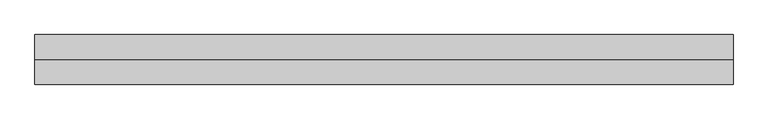
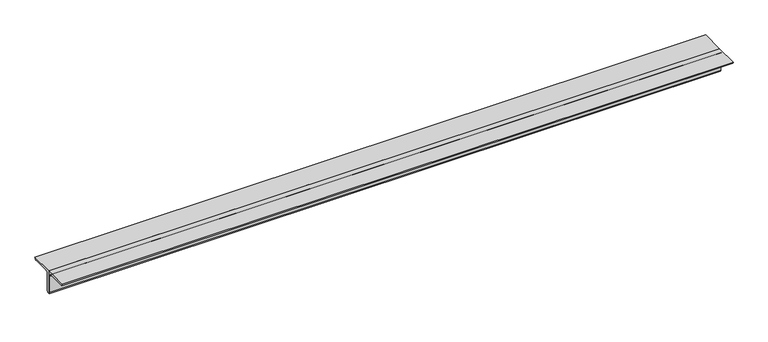
"""IFC4 building model written with IfcOpenShell, lengths in millimetres: member geometry, 0123_Steel Framing_2Ls-KSD3502 : H_SB_AR_S03_2Ls-130x130x12_HBR4."""

import ifcopenshell
import ifcopenshell.guid

model = None  # the IFC model being written
_history = None  # IfcOwnerHistory: only IFC2X3 demands one
_inside = {}  # id of a spatial element -> (the spatial element, [elements in it])
_under = {}  # id of a project, library or spatial element -> (it, [spatial elements below it])
_declared = {}  # id of a project -> (the project, [libraries it declares])
_typed = {}  # id of a type object -> (the type object, [elements of that type])
_made_of = {}  # id of a material, layer set ... -> (it, [elements and type objects made of it])


def new_model(schema):
    """Start an empty IFC model of exactly this schema.

    Asked for "IFC4X3", IfcOpenShell would pick the latest addendum, in which some entities
    have other attributes; the version numbers below select the first issue.
    IFC2X3 requires an IfcOwnerHistory on every rooted entity: one is made here for all.
    """
    global model, _history
    if schema == "IFC4X3":
        model = ifcopenshell.file(schema_version=(4, 3, 0, 0))
    else:
        model = ifcopenshell.file(schema=schema)
    _inside.clear()
    _under.clear()
    _declared.clear()
    _typed.clear()
    _made_of.clear()
    _history = None
    if model.schema == "IFC2X3":
        org = make("IfcOrganization", Name="unknown")
        user = make(
            "IfcPersonAndOrganization",
            ThePerson=make("IfcPerson", FamilyName="unknown"),
            TheOrganization=org,
        )
        app = make(
            "IfcApplication",
            ApplicationDeveloper=org,
            Version="unknown",
            ApplicationFullName="unknown",
            ApplicationIdentifier="unknown",
        )
        _history = make(
            "IfcOwnerHistory",
            OwningUser=user,
            OwningApplication=app,
            ChangeAction="ADDED",
            CreationDate=0,
        )
    return model


def make(cls, **values):
    """One entity of the class cls with the attributes given. An attribute that is None is left unset."""
    return model.create_entity(
        cls, **{name: value for name, value in values.items() if value is not None}
    )


def rooted(cls, **values):
    """An entity with a GlobalId (a new one), such as an element, a storey or a relation."""
    return make(cls, GlobalId=ifcopenshell.guid.new(), OwnerHistory=_history, **values)


def si_unit(unit_type, name, prefix=None):
    """IfcSIUnit, for example si_unit("LENGTHUNIT", "METRE", prefix="MILLI")."""
    return make("IfcSIUnit", UnitType=unit_type, Prefix=prefix, Name=name)


def assignment(units):
    """IfcUnitAssignment: the units of a project."""
    return None if units is None else make("IfcUnitAssignment", Units=units)


def point(xyz):
    """IfcCartesianPoint."""
    return None if xyz is None else make("IfcCartesianPoint", Coordinates=xyz)


def direction(xyz):
    """IfcDirection."""
    return None if xyz is None else make("IfcDirection", DirectionRatios=xyz)


def frame(location, z_axis=None, x_axis=None):
    """IfcAxis2Placement3D, a coordinate frame: its origin and axes. An axis left out is left unset."""
    return make(
        "IfcAxis2Placement3D",
        Location=point(location),
        Axis=direction(z_axis),
        RefDirection=direction(x_axis),
    )


def frame_2d(location, x_axis=None):
    """IfcAxis2Placement2D, a coordinate frame in the plane: its origin and x axis."""
    return make(
        "IfcAxis2Placement2D", Location=point(location), RefDirection=direction(x_axis)
    )


def origin():
    """The frame at (0, 0, 0) with its axes left unset."""
    return frame((0.0, 0.0, 0.0))


def place(relative_to, where):
    """IfcLocalPlacement: puts the frame where relative to a parent placement (None: the world)."""
    return make(
        "IfcLocalPlacement", PlacementRelTo=relative_to, RelativePlacement=where
    )


def context(
    kind, dimensions, precision=None, world=None, true_north=None, identifier=None
):
    """IfcGeometricRepresentationContext, for example the 3D "Model" context."""
    return make(
        "IfcGeometricRepresentationContext",
        ContextIdentifier=identifier,
        ContextType=kind,
        CoordinateSpaceDimension=dimensions,
        Precision=precision,
        WorldCoordinateSystem=world,
        TrueNorth=true_north,
    )


def project(units=None, contexts=None):
    """IfcProject with its units and contexts."""
    return rooted(
        "IfcProject",
        Name="project",
        RepresentationContexts=contexts,
        UnitsInContext=assignment(units),
    )


def spatial(cls, under=None, at=None, **own):
    """A site, building, storey or space (cls), placed at a placement, below another one or the project."""
    s = rooted(cls, ObjectPlacement=at, **own)
    if under is not None:
        _under.setdefault(under.id(), (under, []))[1].append(s)
    return s


def polyline(points):
    """IfcPolyline through the points."""
    return make("IfcPolyline", Points=[point(p) for p in points])


def circle_curve(where, radius):
    """IfcCircle in the frame where."""
    return make("IfcCircle", Position=where, Radius=radius)


def trimmed(basis, trim1, trim2, sense, master):
    """IfcTrimmedCurve: the piece of a basis curve between two trims."""
    return make(
        "IfcTrimmedCurve",
        BasisCurve=basis,
        Trim1=trim1,
        Trim2=trim2,
        SenseAgreement=sense,
        MasterRepresentation=master,
    )


def segment(curve, same_sense, transition):
    """IfcCompositeCurveSegment."""
    return make(
        "IfcCompositeCurveSegment",
        Transition=transition,
        SameSense=same_sense,
        ParentCurve=curve,
    )


def composite_curve(segments, self_intersect=None):
    """IfcCompositeCurve: segments joined end to end."""
    return make("IfcCompositeCurve", Segments=segments, SelfIntersect=self_intersect)


def outline(outer, holes=None, kind="AREA"):
    """IfcArbitraryClosedProfileDef: a profile drawn as a closed curve; with holes, ...WithVoids."""
    if holes is None:
        return make("IfcArbitraryClosedProfileDef", ProfileType=kind, OuterCurve=outer)
    return make(
        "IfcArbitraryProfileDefWithVoids",
        ProfileType=kind,
        OuterCurve=outer,
        InnerCurves=holes,
    )


def extrude(swept, where, along, depth):
    """IfcExtrudedAreaSolid: the profile swept, set in the frame where, extruded along a direction by depth."""
    return make(
        "IfcExtrudedAreaSolid",
        SweptArea=swept,
        Position=where,
        ExtrudedDirection=direction(along),
        Depth=depth,
    )


def shape(context_of_items, identifier, shape_type, items):
    """IfcShapeRepresentation: the items that make up one representation, for example the "Body"."""
    return make(
        "IfcShapeRepresentation",
        ContextOfItems=context_of_items,
        RepresentationIdentifier=identifier,
        RepresentationType=shape_type,
        Items=items,
    )


def source(mapping_origin, context_of_items, identifier, shape_type, items):
    """IfcRepresentationMap: a shape defined once, which mapped items show again and again."""
    return make(
        "IfcRepresentationMap",
        MappingOrigin=mapping_origin,
        MappedRepresentation=shape(context_of_items, identifier, shape_type, items),
    )


def transform(
    local_origin,
    x_axis=None,
    y_axis=None,
    z_axis=None,
    scale=None,
    scale2=None,
    scale3=None,
    uniform=True,
):
    """IfcCartesianTransformationOperator3D, or its non-uniform kind. x_axis, y_axis, z_axis: its Axis1, 2, 3."""
    if uniform:
        return make(
            "IfcCartesianTransformationOperator3D",
            Axis1=direction(x_axis),
            Axis2=direction(y_axis),
            LocalOrigin=point(local_origin),
            Scale=scale,
            Axis3=direction(z_axis),
        )
    return make(
        "IfcCartesianTransformationOperator3DnonUniform",
        Axis1=direction(x_axis),
        Axis2=direction(y_axis),
        LocalOrigin=point(local_origin),
        Scale=scale,
        Axis3=direction(z_axis),
        Scale2=scale2,
        Scale3=scale3,
    )


def mapped(mapping_source, mapping_target):
    """IfcMappedItem: shows the shape of a source again, moved by a transform."""
    return make(
        "IfcMappedItem", MappingSource=mapping_source, MappingTarget=mapping_target
    )


def made_of(thing, what):
    """Note that an element or type object is made of a material, layer set ...; save() writes the relation."""
    if what is not None:
        _made_of.setdefault(what.id(), (what, []))[1].append(thing)
    return thing


def element(
    cls,
    number,
    at=None,
    inside=None,
    cuts=None,
    type_object=None,
    material=None,
    context=None,
    identifier="Body",
    shape_type=None,
    held_by="IfcProductDefinitionShape",
    body=None,
    shapes=None,
    **own,
):
    """One element of the class cls, such as IfcWall. Its Tag is "e" and its number.

    at: its placement. inside: the storey or other place that contains it. cuts: it is an
    opening in that element (IfcRelVoidsElement). A single representation is given by context,
    identifier, shape_type and body (its items); several are given by shapes. held_by: the class
    of the entity that holds the representations. save() writes the other relations.
    """
    e = rooted(cls, Tag="e%d" % number, ObjectPlacement=at, **own)
    if body is not None:
        shapes = [shape(context, identifier, shape_type, body)]
    if shapes is not None:
        e.Representation = make(held_by, Representations=shapes)
    if inside is not None:
        _inside.setdefault(inside.id(), (inside, []))[1].append(e)
    if cuts is not None:
        rooted(
            "IfcRelVoidsElement", RelatingBuildingElement=cuts, RelatedOpeningElement=e
        )
    if type_object is not None:
        _typed.setdefault(type_object.id(), (type_object, []))[1].append(e)
    return made_of(e, material)


def aggregate(whole, parts):
    """IfcRelAggregates: a whole, such as a stair, and the parts it consists of."""
    return rooted("IfcRelAggregates", RelatingObject=whole, RelatedObjects=parts)


def save(model, path):
    """Write the relations noted so far, then the file.

    IfcRelAggregates (storeys below a building ...), IfcRelContainedInSpatialStructure (elements
    in a storey), IfcRelDefinesByType, IfcRelAssociatesMaterial and IfcRelDeclares: one each for
    every whole, place, type object, material and project.
    """
    for whole, parts in _under.values():
        aggregate(whole, parts)
    for where, things in _inside.values():
        rooted(
            "IfcRelContainedInSpatialStructure",
            RelatedElements=things,
            RelatingStructure=where,
        )
    for kind, things in _typed.values():
        rooted("IfcRelDefinesByType", RelatedObjects=things, RelatingType=kind)
    for what, things in _made_of.values():
        rooted("IfcRelAssociatesMaterial", RelatedObjects=things, RelatingMaterial=what)
    for by, libraries in _declared.values():
        rooted("IfcRelDeclares", RelatingContext=by, RelatedDefinitions=libraries)
    model.write(path)


def member_ff9c955f(model_context):
    return source(origin(), model_context, "Body", "SweptSolid", [
        extrude(outline(composite_curve([segment(polyline([(0.0, 36.4), (130.0, 36.4)]), True, "CONTINUOUS"), segment(trimmed(circle_curve(frame_2d((118.0, 36.4)), 12.0), [point((130.0, 36.4))], [point((118.0, 24.4))], False, "CARTESIAN"), True, "CONTINUOUS"), segment(polyline([(118.0, 24.4), (24.0, 24.4)]), True, "CONTINUOUS"), segment(trimmed(circle_curve(frame_2d((24.0, 12.4)), 12.0), [point((24.0, 24.4))], [point((12.0, 12.4))], True, "CARTESIAN"), True, "CONTINUOUS"), segment(polyline([(12.0, 12.4), (12.0, -81.6)]), True, "CONTINUOUS"), segment(trimmed(circle_curve(frame_2d((0.0, -81.6)), 12.0), [point((12.0, -81.6))], [point((0.0, -93.6))], False, "CARTESIAN"), True, "CONTINUOUS"), segment(polyline([(0.0, -93.6), (0.0, 36.4)]), True, "CONTINUOUS")], self_intersect=False)), frame((-1720.2330278, 0.0, 0.0), z_axis=(1.0, 0.0, 0.0), x_axis=(0.0, 1.0, 0.0)), (0.0, 0.0, 1.0), 3660.0954461),
        extrude(outline(composite_curve([segment(polyline([(0.0, 36.4), (0.0, -93.6)]), True, "CONTINUOUS"), segment(trimmed(circle_curve(frame_2d((0.0, -81.6)), 12.0), [point((0.0, -93.6))], [point((-12.0, -81.6))], False, "CARTESIAN"), True, "CONTINUOUS"), segment(polyline([(-12.0, -81.6), (-12.0, 12.4)]), True, "CONTINUOUS"), segment(trimmed(circle_curve(frame_2d((-24.0, 12.4)), 12.0), [point((-12.0, 12.4))], [point((-24.0, 24.4))], True, "CARTESIAN"), True, "CONTINUOUS"), segment(polyline([(-24.0, 24.4), (-118.0, 24.4)]), True, "CONTINUOUS"), segment(trimmed(circle_curve(frame_2d((-118.0, 36.4)), 12.0), [point((-118.0, 24.4))], [point((-130.0, 36.4))], False, "CARTESIAN"), True, "CONTINUOUS"), segment(polyline([(-130.0, 36.4), (0.0, 36.4)]), True, "CONTINUOUS")], self_intersect=False)), frame((-1720.2330278, 0.0, 0.0), z_axis=(1.0, 0.0, 0.0), x_axis=(0.0, 1.0, 0.0)), (0.0, 0.0, 1.0), 3660.0954461),
    ])


if __name__ == "__main__":
    model = new_model("IFC4")
    model_context = context("Model", 3, world=origin())
    ifc_project = project(units=[si_unit("LENGTHUNIT", "METRE", prefix="MILLI")], contexts=[model_context])
    site = spatial("IfcSite", under=ifc_project)
    building = spatial("IfcBuilding", under=site)
    placement = place(None, origin())
    member_shape = member_ff9c955f(model_context)
    element("IfcMember", 1, ObjectType="0123_Steel Framing_2Ls-KSD3502 : H_SB_AR_S03_2Ls-130x130x12_HBR4", at=placement, inside=building, context=model_context, shape_type="MappedRepresentation", body=[
        mapped(member_shape, transform((0.0, 0.0, 0.0), x_axis=(1.0, 0.0, 0.0), y_axis=(0.0, 1.0, 0.0), z_axis=(0.0, 0.0, 1.0))),
    ])
    save(model, "model.ifc")

# Revit data of these elements
# Type "0123_Steel Framing_2Ls-KSD3502 : H_SB_AR_S03_2Ls-130x130x12_HBR4"
#   Type Mark = "HBR4"
#   Assembly Code = "B10"
#   Legs = "SLBB"
#   W = 8.97
#   Perimeter = 1.04 m²/m
#   Nominal Weight = 46.80 kgf/m
#   Length [instance default] = 1000 mm
#   Space = 0 mm
#   b = 130 mm
#   d = 130 mm
#   t = 12 mm
#   y = 36.4 mm
#   A = 0.005952 m²
#   Structural Material [instance default] = Steel ASTM A36
# Element 1 (IfcMember, "0123_Steel Framing_2Ls-KSD3502 : H_SB_AR_S03_2Ls-130x130x12_HBR4")
#   Materials on its faces: "Steel ASTM A36"
# Materials
#   "Steel ASTM A36": class "Metal", colour RGB 199 199 199, transparency 0, Description = "Structural steel, ASTM A36 Grade B, mill finish", Cost = 0
